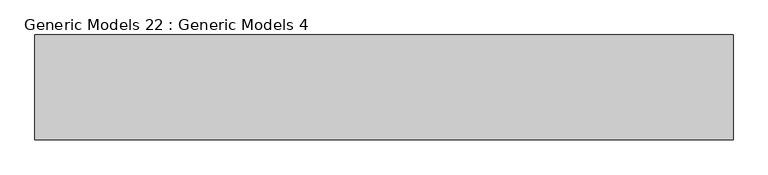
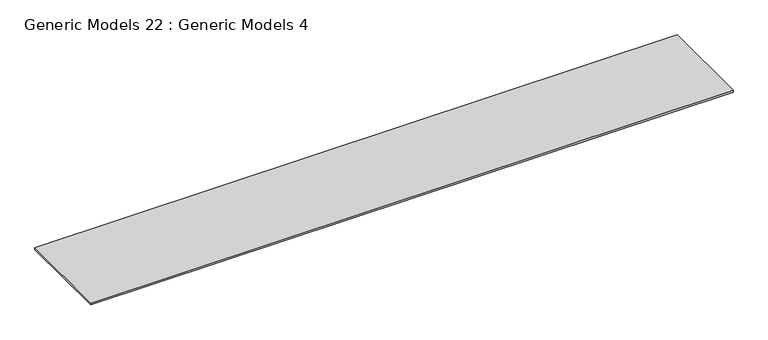
"""IFC4 building model written with IfcOpenShell, lengths in millimetres: proxy geometry, Generic Models 22 : Generic Models 4."""

from ifc_helpers import new_model, si_unit, frame, origin, place, context, project, spatial, polyline, outline, extrude, source, transform, mapped, element, save


def generic_models_22_generic_models_4_18964c74(model_context):
    return source(origin(), model_context, "Body", "SweptSolid", [
        extrude(outline(polyline([(-2152.1733045, -29686.8057997), (-2152.1733045, -30617.9735041), (-8342.1048025, -30617.9735041), (-8342.1048025, -29686.8057997), (-2152.1733045, -29686.8057997)])), frame((0.0, 0.0, 126809.246), z_axis=(0.0, 0.0, 1.0), x_axis=(1.0, 0.0, 0.0)), (0.0, 0.0, 1.0), 19.05),
    ])


if __name__ == "__main__":
    model = new_model("IFC4")
    model_context = context("Model", 3, world=origin())
    ifc_project = project(units=[si_unit("LENGTHUNIT", "METRE", prefix="MILLI")], contexts=[model_context])
    site = spatial("IfcSite", under=ifc_project)
    building = spatial("IfcBuilding", under=site)
    placement = place(None, origin())
    generic_models_22_generic_models_4_shape = generic_models_22_generic_models_4_18964c74(model_context)
    element("IfcBuildingElementProxy", 1, Name="Generic Models 22 : Generic Models 4", ObjectType="Generic Models 22 : Generic Models 4", at=placement, inside=building, context=model_context, shape_type="MappedRepresentation", body=[
        mapped(generic_models_22_generic_models_4_shape, transform((0.0, 0.0, 0.0), x_axis=(1.0, 0.0, 0.0), y_axis=(0.0, 1.0, 0.0), z_axis=(0.0, 0.0, 1.0))),
    ])
    save(model, "model.ifc")

# Revit data of these elements
# Element 1 (IfcBuildingElementProxy, "Generic Models 22 : Generic Models 4")
#   Materials on its faces: "_CDX PLYWOOD - SEE STRUCT DWGs"
# Materials
#   "_CDX PLYWOOD - SEE STRUCT DWGs": class "Generic", colour RGB 98 75 74, transparency 0, Cost = 0
